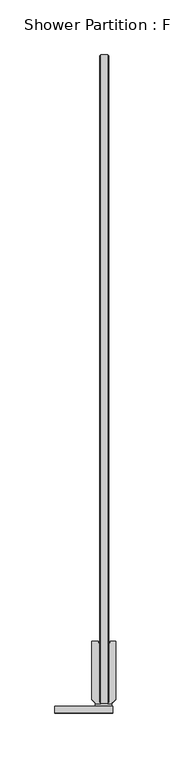
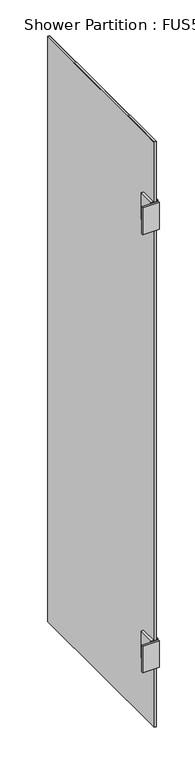
"""IFC4 building model written with IfcOpenShell, lengths in millimetres: furniture geometry, Shower Partition : FUS501_Shower Partition."""

from ifc_helpers import new_model, si_unit, origin, place, context, project, spatial, faceted_brep, source, transform, mapped, element, save


def shower_partition_fus501_shower_partition_aa17ee34(model_context):
    return source(origin(), model_context, "Body", "Brep", [
        faceted_brep([(17.0, -294.0, 1761.208438), (17.0, -291.5, 1761.208438), (13.0420514, -291.5, 1761.208438), (6.9579486, -291.5, 1761.208438), (2.0, -291.5, 1761.208438), (2.0, -294.0, 1761.208438), (17.0, -291.5, 1785.5), (13.0420514, -291.5, 1785.5), (6.9579486, -291.5, 1785.5), (2.0, -291.5, 1785.5), (2.0, -291.5, 1713.920216), (2.0, -291.5, 1694.5), (6.9579486, -291.5, 1694.5), (6.9579486, -291.5, 1713.920216), (13.0420514, -291.5, 1713.920216), (13.0420514, -291.5, 1694.5), (17.0, -291.5, 1694.5), (17.0, -291.5, 1713.920216), (2.0, -294.0, 1713.920216), (17.0, -294.0, 1713.920216), (2.0, -290.5420514, 1785.5), (6.0, -290.5420514, 1785.5), (6.0, -236.5, 1785.5), (4.5, -236.5, 1785.5), (4.5, -234.5, 1785.5), (-1.5, -234.5, 1785.5), (-1.5, -287.828945, 1785.5), (1.2131065, -290.5420514, 1785.5), (17.0, -290.5420514, 1785.5), (17.7868935, -290.5420514, 1785.5), (20.5, -287.828945, 1785.5), (20.5, -234.5, 1785.5), (15.5, -234.5, 1785.5), (15.5, -236.5, 1785.5), (14.0, -236.5, 1785.5), (14.0, -290.5420514, 1785.5), (-35.0, -294.0, 1785.5), (-35.0, -300.0, 1785.5), (17.8567847, -300.0, 1785.5), (17.8567847, -294.0, 1785.5), (17.0, -290.5420514, 1694.5), (14.0, -290.5420514, 1694.5), (14.0, -236.5, 1694.5), (15.5, -236.5, 1694.5), (15.5, -234.5, 1694.5), (20.5, -234.5, 1694.5), (20.5, -287.828945, 1694.5), (17.7868935, -290.5420514, 1694.5), (2.0, -290.5420514, 1694.5), (1.2131065, -290.5420514, 1694.5), (-1.5, -287.828945, 1694.5), (-1.5, -234.5, 1694.5), (4.5, -234.5, 1694.5), (4.5, -236.5, 1694.5), (6.0, -236.5, 1694.5), (6.0, -290.5420514, 1694.5), (17.8567847, -294.0, 1694.5), (17.8567847, -300.0, 1694.5), (-35.0, -300.0, 1694.5), (-35.0, -294.0, 1694.5)], [[[0, 1, 2, 3, 4, 5]], [[1, 6, 7, 2]], [[3, 8, 9, 4]], [[10, 11, 12, 13]], [[14, 15, 16, 17]], [[18, 10, 13, 14, 17, 19]], [[20, 9, 8, 21, 22, 23, 24, 25, 26, 27]], [[7, 6, 28, 29, 30, 31, 32, 33, 34, 35]], [[36, 37, 38, 39]], [[40, 16, 15, 41, 42, 43, 44, 45, 46, 47]], [[12, 11, 48, 49, 50, 51, 52, 53, 54, 55]], [[56, 57, 58, 59]], [[36, 39, 56, 59], [5, 18, 19, 0]], [[48, 11, 10, 18, 5, 4, 9, 20]], [[27, 49, 48, 20]], [[26, 50, 49, 27]], [[25, 51, 50, 26]], [[24, 52, 51, 25]], [[23, 53, 52, 24]], [[34, 42, 41, 35]], [[33, 43, 42, 34]], [[32, 44, 43, 33]], [[31, 45, 44, 32]], [[30, 46, 45, 31]], [[29, 47, 46, 30]], [[28, 40, 47, 29]], [[28, 6, 1, 0, 19, 17, 16, 40]], [[38, 57, 56, 39]], [[37, 58, 57, 38]], [[36, 59, 58, 37]], [[22, 54, 53, 23]], [[21, 55, 54, 22]], [[8, 3, 13, 12, 55, 21]], [[3, 2, 14, 13]], [[35, 41, 15, 14, 2, 7]]]),
        faceted_brep([(2.0, -290.5420514, 295.5), (2.0, -291.5, 295.5), (6.9579486, -291.5, 295.5), (6.0, -290.5420514, 295.5), (6.0, -236.5, 295.5), (4.5, -236.5, 295.5), (4.5, -234.5, 295.5), (-1.5, -234.5, 295.5), (-1.5, -287.828945, 295.5), (1.2131065, -290.5420514, 295.5), (13.0420514, -291.5, 295.5), (17.0, -291.5, 295.5), (17.0, -290.5420514, 295.5), (17.7868935, -290.5420514, 295.5), (20.5, -287.828945, 295.5), (20.5, -234.5, 295.5), (15.5, -234.5, 295.5), (15.5, -236.5, 295.5), (14.0, -236.5, 295.5), (14.0, -290.5420514, 295.5), (-35.0, -294.0, 295.5), (-35.0, -300.0, 295.5), (17.8567847, -300.0, 295.5), (17.8567847, -294.0, 295.5), (17.0, -290.5420514, 204.5), (17.0, -291.5, 204.5), (13.0420514, -291.5, 204.5), (14.0, -290.5420514, 204.5), (14.0, -236.5, 204.5), (15.5, -236.5, 204.5), (15.5, -234.5, 204.5), (20.5, -234.5, 204.5), (20.5, -287.828945, 204.5), (17.7868935, -290.5420514, 204.5), (6.9579486, -291.5, 204.5), (2.0, -291.5, 204.5), (2.0, -290.5420514, 204.5), (1.2131065, -290.5420514, 204.5), (-1.5, -287.828945, 204.5), (-1.5, -234.5, 204.5), (4.5, -234.5, 204.5), (4.5, -236.5, 204.5), (6.0, -236.5, 204.5), (6.0, -290.5420514, 204.5), (17.8567847, -294.0, 204.5), (17.8567847, -300.0, 204.5), (-35.0, -300.0, 204.5), (-35.0, -294.0, 204.5), (2.0, -294.0, 276.079784), (2.0, -294.0, 226.670216), (17.0, -294.0, 226.670216), (17.0, -294.0, 276.079784), (2.0, -291.5, 226.670216), (2.0, -291.5, 276.079784), (17.0, -291.5, 276.079784), (17.0, -291.5, 226.670216), (13.0420514, -291.5, 276.079784), (6.9579486, -291.5, 276.079784), (6.9579486, -291.5, 226.670216), (13.0420514, -291.5, 226.670216)], [[[0, 1, 2, 3, 4, 5, 6, 7, 8, 9]], [[10, 11, 12, 13, 14, 15, 16, 17, 18, 19]], [[20, 21, 22, 23]], [[24, 25, 26, 27, 28, 29, 30, 31, 32, 33]], [[34, 35, 36, 37, 38, 39, 40, 41, 42, 43]], [[44, 45, 46, 47]], [[20, 23, 44, 47], [48, 49, 50, 51]], [[36, 35, 52, 49, 48, 53, 1, 0]], [[9, 37, 36, 0]], [[8, 38, 37, 9]], [[7, 39, 38, 8]], [[6, 40, 39, 7]], [[5, 41, 40, 6]], [[18, 28, 27, 19]], [[17, 29, 28, 18]], [[16, 30, 29, 17]], [[15, 31, 30, 16]], [[14, 32, 31, 15]], [[13, 33, 32, 14]], [[12, 24, 33, 13]], [[12, 11, 54, 51, 50, 55, 25, 24]], [[22, 45, 44, 23]], [[21, 46, 45, 22]], [[20, 47, 46, 21]], [[51, 54, 56, 57, 53, 48]], [[54, 11, 10, 56]], [[57, 2, 1, 53]], [[52, 35, 34, 58]], [[59, 26, 25, 55]], [[49, 52, 58, 59, 55, 50]], [[4, 42, 41, 5]], [[3, 43, 42, 4]], [[2, 57, 58, 34, 43, 3]], [[57, 56, 59, 58]], [[19, 27, 26, 59, 56, 10]]]),
        faceted_brep([(13.0420514, 300.0, 0.0), (13.0420514, -291.5, 0.0), (6.9579486, -291.5, 0.0), (6.9579486, 300.0, 0.0), (13.0420514, -291.5, 1990.0), (13.0420514, 300.0, 1990.0), (6.9579486, 300.0, 1990.0), (6.9579486, -291.5, 1990.0), (6.0, 299.0420514, 0.9579486), (6.0, -290.5420514, 0.9579486), (6.0, -290.5420514, 1989.0420514), (6.0, 299.0420514, 1989.0420514), (14.0, 299.0420514, 1989.0420514), (14.0, -290.5420514, 1989.0420514), (14.0, -290.5420514, 0.9579486), (14.0, 299.0420514, 0.9579486)], [[[0, 1, 2, 3]], [[4, 5, 6, 7]], [[3, 6, 5, 0]], [[8, 9, 10, 11]], [[1, 4, 7, 2]], [[12, 13, 14, 15]], [[8, 11, 6, 3]], [[3, 2, 9, 8]], [[2, 7, 10, 9]], [[11, 10, 7, 6]], [[0, 5, 12, 15]], [[15, 14, 1, 0]], [[14, 13, 4, 1]], [[5, 4, 13, 12]]]),
    ])


if __name__ == "__main__":
    model = new_model("IFC4")
    model_context = context("Model", 3, world=origin())
    ifc_project = project(units=[si_unit("LENGTHUNIT", "METRE", prefix="MILLI")], contexts=[model_context])
    site = spatial("IfcSite", under=ifc_project)
    building = spatial("IfcBuilding", under=site)
    placement = place(None, origin())
    shower_partition_fus501_shower_partition_shape = shower_partition_fus501_shower_partition_aa17ee34(model_context)
    element("IfcFurniture", 1, ObjectType="Shower Partition : FUS501_Shower Partition", at=placement, inside=building, context=model_context, shape_type="MappedRepresentation", body=[
        mapped(shower_partition_fus501_shower_partition_shape, transform((0.0, 0.0, 0.0), x_axis=(1.0, 0.0, 0.0), y_axis=(0.0, 1.0, 0.0), z_axis=(0.0, 0.0, 1.0))),
    ])
    save(model, "model.ifc")

# Revit data of these elements
# Type "Shower Partition : FUS501_Shower Partition"
#   Youtube clip = ""
#   Weight Net (Kg) = "0"
#   Weight = ""
#   WarrantyStartDate [instance default] = "n/a"
#   WarrantyGuarantorParts = "n/a"
#   WarrantyGuarantorLabor = "n/a"
#   WarrantyDurationUnit = "Year"
#   WarrantyDurationParts = "n/a"
#   WarrantyDurationLabor = "n/a"
#   WarrantyDescription = "n/a"
#   VersionDate = "03/02/2020"
#   Version = "1"
#   Uniformat II Description = ""
#   Uniformat II Code = ""
#   Uniclass2015Reference = "Pr_40_20_06_79"
#   Uniclass2015Description = "Shower enclosures"
#   Uniclass2 = "Pr_40_30_06_79"
#   Uniclass 2015 Name = ""
#   Uniclass 2015 Code = ""
#   Uniclass 2.0 Description = ""
#   Uniclass 2.0 Code = ""
#   Uniclass 1.4 Description = ""
#   Uniclass 1.4 Code = ""
#   URL = "https://www.svedbergs.com/products/showers/shower-screen/180-shower-screen-1-door-78-206348/"
#   UNSPSC Code = ""
#   Technical description = ""
#   TagNumber [instance default] = "n/a"
#   SustainabilityPerformance = "n/a"
#   Style = "n/a"
#   Size = "70x780x2000mm"
#   Shape = "Rectangular"
#   SerialNumber [instance default] = "n/a"
#   Revision = "n/a"
#   ReplacementCost = "n/a"
#   Region South America = "All"
#   Region Oceania = "All"
#   Region North America = "All"
#   Region Middle East = "All"
#   Region Europe = "All"
#   Region Asia = "All"
#   Region Antarctica = "All"
#   Region Africa = "All"
#   RSKNumber = "7331415"
#   QR code = "http://bimobject.com/svedbergs/product/shower-78_shower"
#   ProductInformation = "Has one opening door. Doors can be folded inwards when shower is not in use to maximise floor space. No threshold – allows disabled access. Toughened safety glass 8 mm. Self-closing hinges. Concealed mounting & clamping screws. Height 200 cm. Door opening 75-95 cm."
#   ProductDatasheet = "https://www.svedbergs.com/products/showers/shower-screen/180-shower-screen-1-door-78-206348/GetPdf/?code=206348&productName=180%C2%B0%20Shower%20screen%201%20door%2078"
#   Product url = "https://www.svedbergs.com/products/showers/shower-screen/180-shower-screen-1-door-78-206348/"
#   Product group = "Shower Screen"
#   Product family = "180"
#   Product data url = "https://bimobject.com/svedbergs/product/shower-78_shower"
#   Product certification = ""
#   Product SKU = "shower-78_shower"
#   Product Guid = "bad75198-8fba-4d63-8e5f-588e794387c3"
#   OmniClass Description = ""
#   OmniClass Code = ""
#   Name = "180_Shower-screen_78"
#   NBSReference = "45-35-70/332"
#   NBSDescription = "Shower enclosures"
#   NBS Reference Description = ""
#   NBS Reference Code = ""
#   ModelReference = "681778"
#   ModelNumber = "n/a"
#   Material secondary = ""
#   Material main = ""
#   Material = "Glass, metal"
#   Masterformat 2014 Description = ""
#   Masterformat 2014 Code = ""
#   ManufacturerURL = "https://www.svedbergs.com/"
#   ManufacturerName = "Svedbergs"
#   Manufacturer name = ""
#   Manufacturer country = "Sweden"
#   MainColor = "Transparent"
#   InstallationDate [instance default] = "n/a"
#   Installation instructions = ""
#   IFC Classification = ""
#   GTIN code = ""
#   EANNumber = "7323100206787"
#   Design country = "Sweden"
#   Description = "Has one opening door. Doors can be folded inwards when shower is not in use to maximise floor space. No threshold – allows disabled access. Toughened safety glass 8 mm. Self-closing hinges. Concealed mounting & clamping screws. Height 200 cm. Door opening 75-95 cm."
#   Date of publishing = ""
#   Collection = "180°"
#   Model = "180° Shower Door 78 - Chrome/Clear glass"
#   Manufacturer = "Svedbergs"
#   IfcExportType = "NOTDEFINED"
#   IfcExportAs = "IfcFurnitureType"
#   Grade = "n/a"
#   Finish = "Black Mat/Clear glass"
#   Features = "Accessories:Shower seat Relax"
#   ExpectedLife = "n/a"
#   DurationUnit = "Year"
#   ConvergoRefNr = "0056-1912-0096-SE\t\t\r\n"
#   Constituents = "n/a"
#   Color = "Transparent"
#   CodePerformance = "n/a"
#   Category = "Shower screen"
#   COBIe Type Category = ""
#   Brand url = "http://www.svedbergs.com/"
#   Brand = "Svedbergs"
#   Barcode [instance default] = "n/a"
#   BIMobject main category code = "sanitary"
#   BIMobject main category = "Sanitary"
#   BIMobject category code = "sanitary-shower-screens"
#   BIMobject category = "Shower screens"
#   BIMObjectName = "Sanitary_Shower-screens_Svedbergs_180_Shower-screen_78"
#   Author = "Convergo AB"
#   AssetType = "Fixed"
#   AssetIdentifier [instance default] = "n/a"
#   AssemblyInstruction = "https://www.svedbergs.com/globalassets/catalog-assets/documentfile/99248-M1_180_dorr.pdf"
#   AccessibilityPerformance = "n/a"
#   NominalLength = 70 mm
#   NominalDepth = 600 mm
#   Nominal width = 0 mm
#   Nominal height = 0 mm
#   Edition number = 1
#   ShowerEnclosureSecondaryMaterial = Black Mat
#   ShowerEnclosureMainMaterial = Clear Glass
#   Type Comments = ""
#   Default Elevation = 0
#   Cost = 0
# Element 1 (IfcFurniture, "Shower Partition : FUS501_Shower Partition")
#   Materials on its faces: "Black Mat", "Clear Glass"
# Materials
#   "Black Mat": class "Metal", colour RGB 20 20 20, transparency 0, Cost = 0
#   "Clear Glass": class "Glass", colour RGB 236 240 239, transparency 0.85, Description = "Clear glazing", Cost = 0
